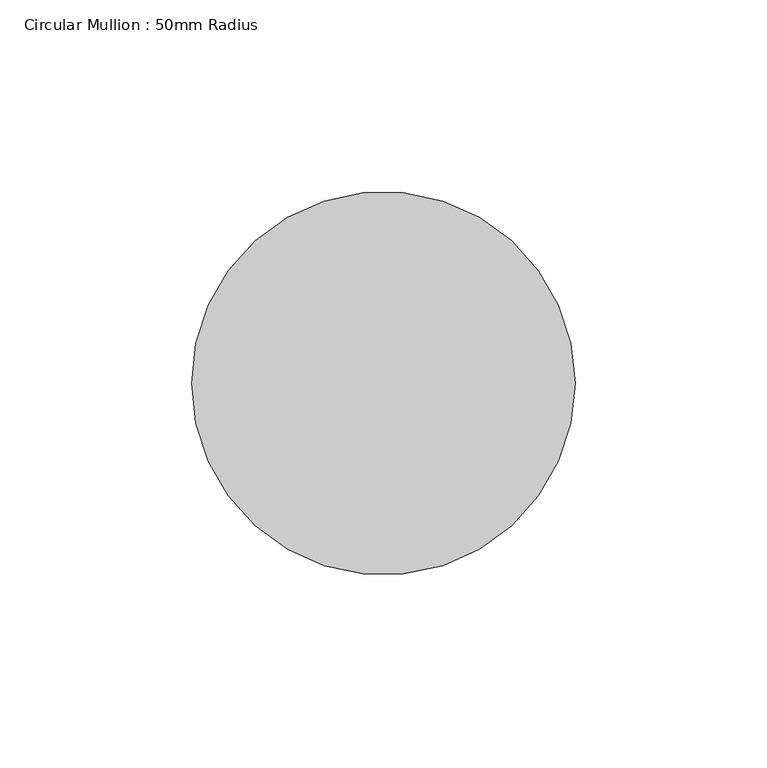
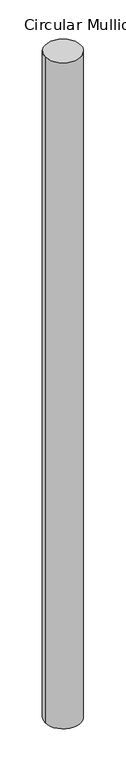
"""IFC4 building model written with IfcOpenShell, lengths in millimetres: member geometry, Circular Mullion : 50mm Radius."""

from ifc_helpers import new_model, si_unit, point, frame, origin, origin_2d, place, context, project, spatial, circle_curve, trimmed, segment, composite_curve, outline, extrude, source, transform, mapped, element, save


def circular_mullion_50mm_radius_47caaa2d(model_context):
    return source(origin(), model_context, "Body", "SweptSolid", [
        extrude(outline(composite_curve([segment(trimmed(circle_curve(origin_2d(), 50.0), [point((50.0, 0.0))], [point((-50.0, 0.0))], False, "CARTESIAN"), True, "CONTINUOUS"), segment(trimmed(circle_curve(origin_2d(), 50.0), [point((-50.0, 0.0))], [point((50.0, 0.0))], False, "CARTESIAN"), True, "CONTINUOUS")], self_intersect=False)), frame((0.0, 0.0, -1977.8023807), z_axis=(0.0, 0.0, 1.0), x_axis=(1.0, 0.0, 0.0)), (0.0, 0.0, 1.0), 1977.8023807),
    ])


if __name__ == "__main__":
    model = new_model("IFC4")
    model_context = context("Model", 3, world=origin())
    ifc_project = project(units=[si_unit("LENGTHUNIT", "METRE", prefix="MILLI")], contexts=[model_context])
    site = spatial("IfcSite", under=ifc_project)
    building = spatial("IfcBuilding", under=site)
    placement = place(None, origin())
    circular_mullion_50mm_radius_shape = circular_mullion_50mm_radius_47caaa2d(model_context)
    element("IfcMember", 1, ObjectType="Circular Mullion : 50mm Radius", at=placement, inside=building, context=model_context, shape_type="MappedRepresentation", body=[
        mapped(circular_mullion_50mm_radius_shape, transform((0.0, 0.0, 0.0), x_axis=(1.0, 0.0, 0.0), y_axis=(0.0, 1.0, 0.0), z_axis=(0.0, 0.0, 1.0))),
    ])
    save(model, "model.ifc")

# Revit data of these elements
# Type "Circular Mullion : 50mm Radius"
#   built-in parameter 1007350 = 0.164042 (stored number, unit not read)
# Element 1 (IfcMember, "Circular Mullion : 50mm Radius")
#   Materials on its faces: "Aluminium"
# Materials
#   "Aluminium": class "Metal", colour RGB 247 247 247, transparency 0, Description = "Aluminium 6061", Cost = 0
